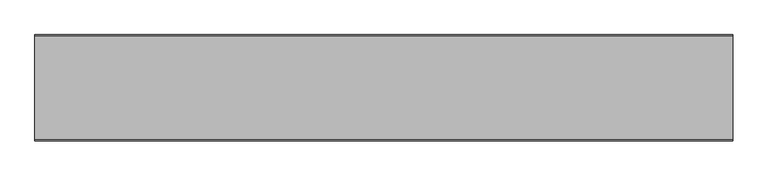
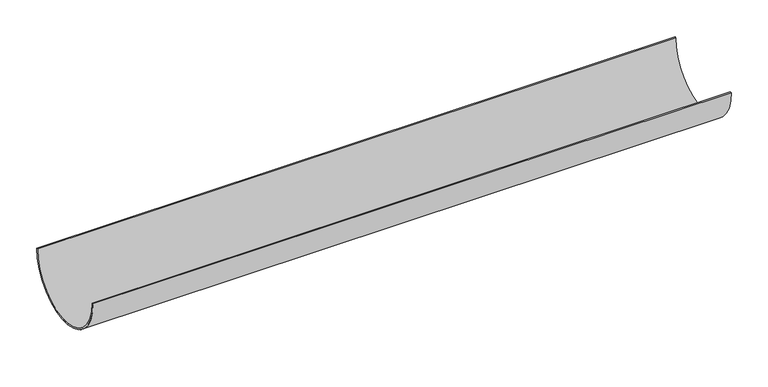
"""IFC4 building model written with IfcOpenShell, lengths in millimetres: proxy geometry, TN_ПВС 125-82_Водосточный желоб : TN_ПВС 125-82_Водосточный желоб."""

from ifc_helpers import new_model, si_unit, point, frame, origin, origin_2d, place, context, project, spatial, polyline, circle_curve, trimmed, segment, composite_curve, outline, extrude, source, transform, mapped, element, save


def generic_models_29262e14(model_context):
    return source(origin(), model_context, "Body", "SweptSolid", [
        extrude(outline(composite_curve([segment(trimmed(circle_curve(origin_2d(), 76.1), [point((76.1, 0.0))], [point((-76.1, 0.0))], False, "CARTESIAN"), True, "CONTINUOUS"), segment(polyline([(-76.1, 0.0), (-74.1, 0.0)]), True, "CONTINUOUS"), segment(trimmed(circle_curve(origin_2d(), 74.1), [point((-74.1, 0.0))], [point((74.1, 0.0))], True, "CARTESIAN"), True, "CONTINUOUS"), segment(polyline([(74.1, 0.0), (76.1, 0.0)]), True, "CONTINUOUS")], self_intersect=False)), frame((0.0, 0.0, 0.0), z_axis=(1.0, 0.0, 0.0), x_axis=(0.0, 1.0, 0.0)), (0.0, 0.0, 1.0), 1000.0),
    ])


if __name__ == "__main__":
    model = new_model("IFC4")
    model_context = context("Model", 3, world=origin())
    ifc_project = project(units=[si_unit("LENGTHUNIT", "METRE", prefix="MILLI")], contexts=[model_context])
    site = spatial("IfcSite", under=ifc_project)
    building = spatial("IfcBuilding", under=site)
    placement = place(None, origin())
    generic_models_shape = generic_models_29262e14(model_context)
    element("IfcBuildingElementProxy", 1, Name="TN_ПВС 125-82_Водосточный желоб : TN_ПВС 125-82_Водосточный желоб", ObjectType="TN_ПВС 125-82_Водосточный желоб : TN_ПВС 125-82_Водосточный желоб", at=placement, inside=building, context=model_context, shape_type="MappedRepresentation", body=[
        mapped(generic_models_shape, transform((0.0, 0.0, 0.0), x_axis=(1.0, 0.0, 0.0), y_axis=(0.0, 1.0, 0.0), z_axis=(0.0, 0.0, 1.0))),
    ])
    save(model, "model.ifc")

# Revit data of these elements
# Type "TN_ПВС 125-82_Водосточный желоб : TN_ПВС 125-82_Водосточный желоб"
#   Description = "Предназначен для сбора дождевой\r\nи талой воды с кровли."
#   Manufacturer = "ТехноНИКОЛЬ"
#   Model = "Комплектующие к водосточным системам"
#   URL = "https://tn-vodostok.ru/catalog/pvh/"
#   ADSK_Обозначение = "ТехноНИКОЛЬ"
#   ADSK_Наименование краткое = "Желоб"
#   ADSK_Наименование = "Водосточный желоб"
#   ADSK_Масса_Текст = ""
#   ADSK_Марка = ""
#   ADSK_Код изделия = ""
#   ADSK_Завод-изготовитель = "ТехноНИКОЛЬ"
#   ADSK_Единица измерения = "п.м."
#   ADSK_Группирование = "Комплектующие к водосточным системам"
#   ADSK_URL страницы изделия = "https://tn-vodostok.ru/catalog/pvh/"
#   ADSK_URL документации изделия = "https://tn-vodostok.ru/upload/iblock/c42/c427963cb77eb5c3c51f0cfb870e9e52.pdf"
#   ADSK_Размер_Длина [instance default] = 500 mm
#   ADSK_Количество [instance default] = 0.5
#   ADSK_Материал [instance default] = TN_Пластик_Коричневый_RAL8019
#   Default Elevation = 0
# Element 1 (IfcBuildingElementProxy, "TN_ПВС 125-82_Водосточный желоб : TN_ПВС 125-82_Водосточный желоб")
#   ADSK_Размер_Длина = 1000 mm
#   ADSK_Количество = 1
#   Materials on its faces: "TN_Пластик_Коричневый_RAL8019"
# Materials
#   "TN_Пластик_Коричневый_RAL8019": class "Типовые", colour RGB 61 54 53, transparency 0, Cost = 0
